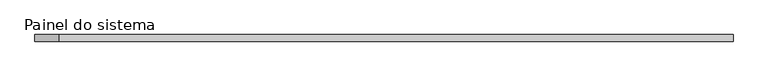
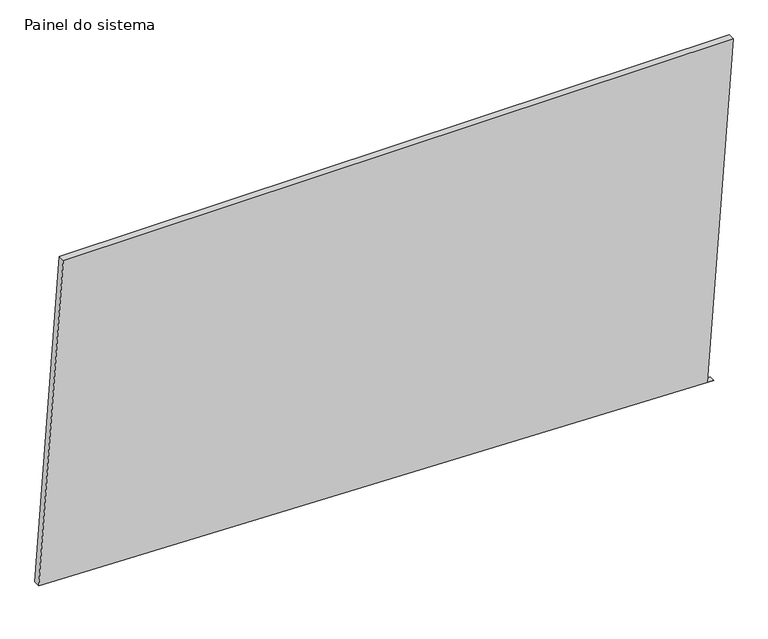
"""IFC4 building model written with IfcOpenShell, lengths in millimetres: plate geometry, Painel do sistema : Envidraçado."""

import ifcopenshell
import ifcopenshell.guid

model = None  # the IFC model being written
_history = None  # IfcOwnerHistory: only IFC2X3 demands one
_inside = {}  # id of a spatial element -> (the spatial element, [elements in it])
_under = {}  # id of a project, library or spatial element -> (it, [spatial elements below it])
_declared = {}  # id of a project -> (the project, [libraries it declares])
_typed = {}  # id of a type object -> (the type object, [elements of that type])
_made_of = {}  # id of a material, layer set ... -> (it, [elements and type objects made of it])


def new_model(schema):
    """Start an empty IFC model of exactly this schema.

    Asked for "IFC4X3", IfcOpenShell would pick the latest addendum, in which some entities
    have other attributes; the version numbers below select the first issue.
    IFC2X3 requires an IfcOwnerHistory on every rooted entity: one is made here for all.
    """
    global model, _history
    if schema == "IFC4X3":
        model = ifcopenshell.file(schema_version=(4, 3, 0, 0))
    else:
        model = ifcopenshell.file(schema=schema)
    _inside.clear()
    _under.clear()
    _declared.clear()
    _typed.clear()
    _made_of.clear()
    _history = None
    if model.schema == "IFC2X3":
        org = make("IfcOrganization", Name="unknown")
        user = make(
            "IfcPersonAndOrganization",
            ThePerson=make("IfcPerson", FamilyName="unknown"),
            TheOrganization=org,
        )
        app = make(
            "IfcApplication",
            ApplicationDeveloper=org,
            Version="unknown",
            ApplicationFullName="unknown",
            ApplicationIdentifier="unknown",
        )
        _history = make(
            "IfcOwnerHistory",
            OwningUser=user,
            OwningApplication=app,
            ChangeAction="ADDED",
            CreationDate=0,
        )
    return model


def make(cls, **values):
    """One entity of the class cls with the attributes given. An attribute that is None is left unset."""
    return model.create_entity(
        cls, **{name: value for name, value in values.items() if value is not None}
    )


def rooted(cls, **values):
    """An entity with a GlobalId (a new one), such as an element, a storey or a relation."""
    return make(cls, GlobalId=ifcopenshell.guid.new(), OwnerHistory=_history, **values)


def si_unit(unit_type, name, prefix=None):
    """IfcSIUnit, for example si_unit("LENGTHUNIT", "METRE", prefix="MILLI")."""
    return make("IfcSIUnit", UnitType=unit_type, Prefix=prefix, Name=name)


def assignment(units):
    """IfcUnitAssignment: the units of a project."""
    return None if units is None else make("IfcUnitAssignment", Units=units)


def point(xyz):
    """IfcCartesianPoint."""
    return None if xyz is None else make("IfcCartesianPoint", Coordinates=xyz)


def direction(xyz):
    """IfcDirection."""
    return None if xyz is None else make("IfcDirection", DirectionRatios=xyz)


def frame(location, z_axis=None, x_axis=None):
    """IfcAxis2Placement3D, a coordinate frame: its origin and axes. An axis left out is left unset."""
    return make(
        "IfcAxis2Placement3D",
        Location=point(location),
        Axis=direction(z_axis),
        RefDirection=direction(x_axis),
    )


def origin():
    """The frame at (0, 0, 0) with its axes left unset."""
    return frame((0.0, 0.0, 0.0))


def place(relative_to, where):
    """IfcLocalPlacement: puts the frame where relative to a parent placement (None: the world)."""
    return make(
        "IfcLocalPlacement", PlacementRelTo=relative_to, RelativePlacement=where
    )


def context(
    kind, dimensions, precision=None, world=None, true_north=None, identifier=None
):
    """IfcGeometricRepresentationContext, for example the 3D "Model" context."""
    return make(
        "IfcGeometricRepresentationContext",
        ContextIdentifier=identifier,
        ContextType=kind,
        CoordinateSpaceDimension=dimensions,
        Precision=precision,
        WorldCoordinateSystem=world,
        TrueNorth=true_north,
    )


def project(units=None, contexts=None):
    """IfcProject with its units and contexts."""
    return rooted(
        "IfcProject",
        Name="project",
        RepresentationContexts=contexts,
        UnitsInContext=assignment(units),
    )


def spatial(cls, under=None, at=None, **own):
    """A site, building, storey or space (cls), placed at a placement, below another one or the project."""
    s = rooted(cls, ObjectPlacement=at, **own)
    if under is not None:
        _under.setdefault(under.id(), (under, []))[1].append(s)
    return s


def polyline(points):
    """IfcPolyline through the points."""
    return make("IfcPolyline", Points=[point(p) for p in points])


def outline(outer, holes=None, kind="AREA"):
    """IfcArbitraryClosedProfileDef: a profile drawn as a closed curve; with holes, ...WithVoids."""
    if holes is None:
        return make("IfcArbitraryClosedProfileDef", ProfileType=kind, OuterCurve=outer)
    return make(
        "IfcArbitraryProfileDefWithVoids",
        ProfileType=kind,
        OuterCurve=outer,
        InnerCurves=holes,
    )


def extrude(swept, where, along, depth):
    """IfcExtrudedAreaSolid: the profile swept, set in the frame where, extruded along a direction by depth."""
    return make(
        "IfcExtrudedAreaSolid",
        SweptArea=swept,
        Position=where,
        ExtrudedDirection=direction(along),
        Depth=depth,
    )


def shape(context_of_items, identifier, shape_type, items):
    """IfcShapeRepresentation: the items that make up one representation, for example the "Body"."""
    return make(
        "IfcShapeRepresentation",
        ContextOfItems=context_of_items,
        RepresentationIdentifier=identifier,
        RepresentationType=shape_type,
        Items=items,
    )


def source(mapping_origin, context_of_items, identifier, shape_type, items):
    """IfcRepresentationMap: a shape defined once, which mapped items show again and again."""
    return make(
        "IfcRepresentationMap",
        MappingOrigin=mapping_origin,
        MappedRepresentation=shape(context_of_items, identifier, shape_type, items),
    )


def transform(
    local_origin,
    x_axis=None,
    y_axis=None,
    z_axis=None,
    scale=None,
    scale2=None,
    scale3=None,
    uniform=True,
):
    """IfcCartesianTransformationOperator3D, or its non-uniform kind. x_axis, y_axis, z_axis: its Axis1, 2, 3."""
    if uniform:
        return make(
            "IfcCartesianTransformationOperator3D",
            Axis1=direction(x_axis),
            Axis2=direction(y_axis),
            LocalOrigin=point(local_origin),
            Scale=scale,
            Axis3=direction(z_axis),
        )
    return make(
        "IfcCartesianTransformationOperator3DnonUniform",
        Axis1=direction(x_axis),
        Axis2=direction(y_axis),
        LocalOrigin=point(local_origin),
        Scale=scale,
        Axis3=direction(z_axis),
        Scale2=scale2,
        Scale3=scale3,
    )


def mapped(mapping_source, mapping_target):
    """IfcMappedItem: shows the shape of a source again, moved by a transform."""
    return make(
        "IfcMappedItem", MappingSource=mapping_source, MappingTarget=mapping_target
    )


def made_of(thing, what):
    """Note that an element or type object is made of a material, layer set ...; save() writes the relation."""
    if what is not None:
        _made_of.setdefault(what.id(), (what, []))[1].append(thing)
    return thing


def element(
    cls,
    number,
    at=None,
    inside=None,
    cuts=None,
    type_object=None,
    material=None,
    context=None,
    identifier="Body",
    shape_type=None,
    held_by="IfcProductDefinitionShape",
    body=None,
    shapes=None,
    **own,
):
    """One element of the class cls, such as IfcWall. Its Tag is "e" and its number.

    at: its placement. inside: the storey or other place that contains it. cuts: it is an
    opening in that element (IfcRelVoidsElement). A single representation is given by context,
    identifier, shape_type and body (its items); several are given by shapes. held_by: the class
    of the entity that holds the representations. save() writes the other relations.
    """
    e = rooted(cls, Tag="e%d" % number, ObjectPlacement=at, **own)
    if body is not None:
        shapes = [shape(context, identifier, shape_type, body)]
    if shapes is not None:
        e.Representation = make(held_by, Representations=shapes)
    if inside is not None:
        _inside.setdefault(inside.id(), (inside, []))[1].append(e)
    if cuts is not None:
        rooted(
            "IfcRelVoidsElement", RelatingBuildingElement=cuts, RelatedOpeningElement=e
        )
    if type_object is not None:
        _typed.setdefault(type_object.id(), (type_object, []))[1].append(e)
    return made_of(e, material)


def aggregate(whole, parts):
    """IfcRelAggregates: a whole, such as a stair, and the parts it consists of."""
    return rooted("IfcRelAggregates", RelatingObject=whole, RelatedObjects=parts)


def save(model, path):
    """Write the relations noted so far, then the file.

    IfcRelAggregates (storeys below a building ...), IfcRelContainedInSpatialStructure (elements
    in a storey), IfcRelDefinesByType, IfcRelAssociatesMaterial and IfcRelDeclares: one each for
    every whole, place, type object, material and project.
    """
    for whole, parts in _under.values():
        aggregate(whole, parts)
    for where, things in _inside.values():
        rooted(
            "IfcRelContainedInSpatialStructure",
            RelatedElements=things,
            RelatingStructure=where,
        )
    for kind, things in _typed.values():
        rooted("IfcRelDefinesByType", RelatedObjects=things, RelatingType=kind)
    for what, things in _made_of.values():
        rooted("IfcRelAssociatesMaterial", RelatedObjects=things, RelatingMaterial=what)
    for by, libraries in _declared.values():
        rooted("IfcRelDeclares", RelatingContext=by, RelatedDefinitions=libraries)
    model.write(path)


def painel_do_sistema_1d411473(model_context):
    return source(origin(), model_context, "Body", "SweptSolid", [
        extrude(outline(polyline([(0.0, 1250.2472418), (1.8159485, 1225.3132824), (1354.0372766, 1323.7960077), (1354.0372766, -1230.5806486), (74.1397484, -1323.7960077), (0.0, 1250.2472418)])), frame((0.0, 24.5, 0.0), z_axis=(0.0, 1.0, 0.0), x_axis=(0.0, 0.0, 1.0)), (0.0, 0.0, 1.0), 25.0),
    ])


if __name__ == "__main__":
    model = new_model("IFC4")
    model_context = context("Model", 3, world=origin())
    ifc_project = project(units=[si_unit("LENGTHUNIT", "METRE", prefix="MILLI")], contexts=[model_context])
    site = spatial("IfcSite", under=ifc_project)
    building = spatial("IfcBuilding", under=site)
    placement = place(None, origin())
    painel_do_sistema_shape = painel_do_sistema_1d411473(model_context)
    element("IfcPlate", 1, ObjectType="Painel do sistema : Envidraçado", at=placement, inside=building, context=model_context, shape_type="MappedRepresentation", body=[
        mapped(painel_do_sistema_shape, transform((0.0, 0.0, 0.0), x_axis=(1.0, 0.0, 0.0), y_axis=(0.0, 1.0, 0.0), z_axis=(0.0, 0.0, 1.0))),
    ])
    save(model, "model.ifc")

# Revit data of these elements
# Type "Painel do sistema : Envidraçado"
#   Construction Type Id = "GSP4R"
#   Analytic Construction = "Vidraça única Pilkington 1/8 pol"
#   Visual Light Transmittance = 0.9
#   Solar Heat Gain Coefficient = 0.86
#   Heat Transfer Coefficient (U) = 6.7069 W/(m²·K)
# Element 1 (IfcPlate, "Painel do sistema : Envidraçado")
#   Materials on its faces: "Vidro"
# Materials
#   "Vidro": class "Vidro", colour RGB 0 128 192, transparency 0.9, Description = "Vidro de sílica", Cost = 0
